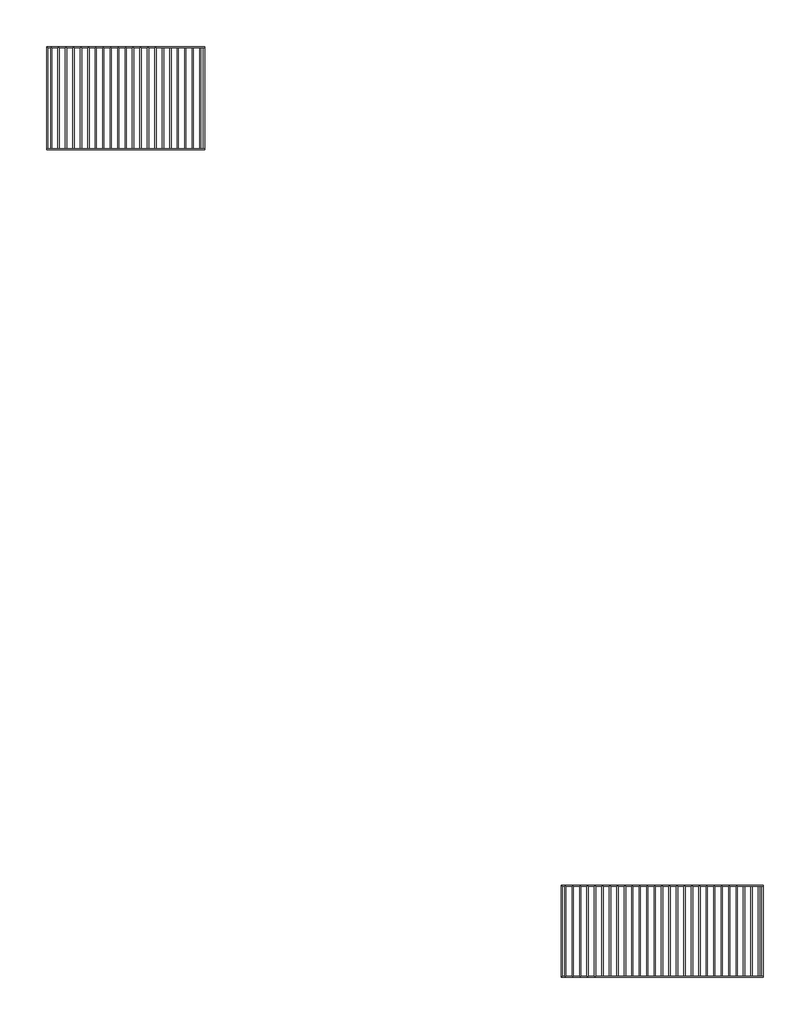
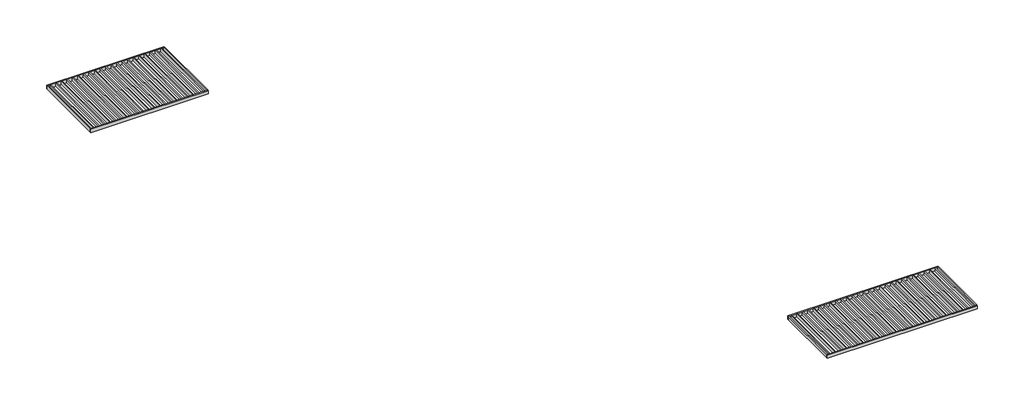
# One storey: 56 beams.
"""IFC4 building model written with IfcOpenShell, lengths in millimetres."""

import ifcopenshell
import ifcopenshell.guid

model = None  # the IFC model being written
_history = None  # IfcOwnerHistory: only IFC2X3 demands one
_inside = {}  # id of a spatial element -> (the spatial element, [elements in it])
_under = {}  # id of a project, library or spatial element -> (it, [spatial elements below it])
_declared = {}  # id of a project -> (the project, [libraries it declares])
_typed = {}  # id of a type object -> (the type object, [elements of that type])
_made_of = {}  # id of a material, layer set ... -> (it, [elements and type objects made of it])


def new_model(schema):
    """Start an empty IFC model of exactly this schema.

    Asked for "IFC4X3", IfcOpenShell would pick the latest addendum, in which some entities
    have other attributes; the version numbers below select the first issue.
    IFC2X3 requires an IfcOwnerHistory on every rooted entity: one is made here for all.
    """
    global model, _history
    if schema == "IFC4X3":
        model = ifcopenshell.file(schema_version=(4, 3, 0, 0))
    else:
        model = ifcopenshell.file(schema=schema)
    _inside.clear()
    _under.clear()
    _declared.clear()
    _typed.clear()
    _made_of.clear()
    _history = None
    if model.schema == "IFC2X3":
        org = make("IfcOrganization", Name="unknown")
        user = make(
            "IfcPersonAndOrganization",
            ThePerson=make("IfcPerson", FamilyName="unknown"),
            TheOrganization=org,
        )
        app = make(
            "IfcApplication",
            ApplicationDeveloper=org,
            Version="unknown",
            ApplicationFullName="unknown",
            ApplicationIdentifier="unknown",
        )
        _history = make(
            "IfcOwnerHistory",
            OwningUser=user,
            OwningApplication=app,
            ChangeAction="ADDED",
            CreationDate=0,
        )
    return model


def make(cls, **values):
    """One entity of the class cls with the attributes given. An attribute that is None is left unset."""
    return model.create_entity(
        cls, **{name: value for name, value in values.items() if value is not None}
    )


def rooted(cls, **values):
    """An entity with a GlobalId (a new one), such as an element, a storey or a relation."""
    return make(cls, GlobalId=ifcopenshell.guid.new(), OwnerHistory=_history, **values)


def si_unit(unit_type, name, prefix=None):
    """IfcSIUnit, for example si_unit("LENGTHUNIT", "METRE", prefix="MILLI")."""
    return make("IfcSIUnit", UnitType=unit_type, Prefix=prefix, Name=name)


def assignment(units):
    """IfcUnitAssignment: the units of a project."""
    return None if units is None else make("IfcUnitAssignment", Units=units)


def point(xyz):
    """IfcCartesianPoint."""
    return None if xyz is None else make("IfcCartesianPoint", Coordinates=xyz)


def direction(xyz):
    """IfcDirection."""
    return None if xyz is None else make("IfcDirection", DirectionRatios=xyz)


def frame(location, z_axis=None, x_axis=None):
    """IfcAxis2Placement3D, a coordinate frame: its origin and axes. An axis left out is left unset."""
    return make(
        "IfcAxis2Placement3D",
        Location=point(location),
        Axis=direction(z_axis),
        RefDirection=direction(x_axis),
    )


def origin():
    """The frame at (0, 0, 0) with its axes left unset."""
    return frame((0.0, 0.0, 0.0))


def place(relative_to, where):
    """IfcLocalPlacement: puts the frame where relative to a parent placement (None: the world)."""
    return make(
        "IfcLocalPlacement", PlacementRelTo=relative_to, RelativePlacement=where
    )


def context(
    kind, dimensions, precision=None, world=None, true_north=None, identifier=None
):
    """IfcGeometricRepresentationContext, for example the 3D "Model" context."""
    return make(
        "IfcGeometricRepresentationContext",
        ContextIdentifier=identifier,
        ContextType=kind,
        CoordinateSpaceDimension=dimensions,
        Precision=precision,
        WorldCoordinateSystem=world,
        TrueNorth=true_north,
    )


def project(units=None, contexts=None):
    """IfcProject with its units and contexts."""
    return rooted(
        "IfcProject",
        Name="project",
        RepresentationContexts=contexts,
        UnitsInContext=assignment(units),
    )


def spatial(cls, under=None, at=None, **own):
    """A site, building, storey or space (cls), placed at a placement, below another one or the project."""
    s = rooted(cls, ObjectPlacement=at, **own)
    if under is not None:
        _under.setdefault(under.id(), (under, []))[1].append(s)
    return s


def polyline(points):
    """IfcPolyline through the points."""
    return make("IfcPolyline", Points=[point(p) for p in points])


def outline(outer, holes=None, kind="AREA"):
    """IfcArbitraryClosedProfileDef: a profile drawn as a closed curve; with holes, ...WithVoids."""
    if holes is None:
        return make("IfcArbitraryClosedProfileDef", ProfileType=kind, OuterCurve=outer)
    return make(
        "IfcArbitraryProfileDefWithVoids",
        ProfileType=kind,
        OuterCurve=outer,
        InnerCurves=holes,
    )


def extrude(swept, where, along, depth):
    """IfcExtrudedAreaSolid: the profile swept, set in the frame where, extruded along a direction by depth."""
    return make(
        "IfcExtrudedAreaSolid",
        SweptArea=swept,
        Position=where,
        ExtrudedDirection=direction(along),
        Depth=depth,
    )


def shape(context_of_items, identifier, shape_type, items):
    """IfcShapeRepresentation: the items that make up one representation, for example the "Body"."""
    return make(
        "IfcShapeRepresentation",
        ContextOfItems=context_of_items,
        RepresentationIdentifier=identifier,
        RepresentationType=shape_type,
        Items=items,
    )


def source(mapping_origin, context_of_items, identifier, shape_type, items):
    """IfcRepresentationMap: a shape defined once, which mapped items show again and again."""
    return make(
        "IfcRepresentationMap",
        MappingOrigin=mapping_origin,
        MappedRepresentation=shape(context_of_items, identifier, shape_type, items),
    )


def transform(
    local_origin,
    x_axis=None,
    y_axis=None,
    z_axis=None,
    scale=None,
    scale2=None,
    scale3=None,
    uniform=True,
):
    """IfcCartesianTransformationOperator3D, or its non-uniform kind. x_axis, y_axis, z_axis: its Axis1, 2, 3."""
    if uniform:
        return make(
            "IfcCartesianTransformationOperator3D",
            Axis1=direction(x_axis),
            Axis2=direction(y_axis),
            LocalOrigin=point(local_origin),
            Scale=scale,
            Axis3=direction(z_axis),
        )
    return make(
        "IfcCartesianTransformationOperator3DnonUniform",
        Axis1=direction(x_axis),
        Axis2=direction(y_axis),
        LocalOrigin=point(local_origin),
        Scale=scale,
        Axis3=direction(z_axis),
        Scale2=scale2,
        Scale3=scale3,
    )


def mapped(mapping_source, mapping_target):
    """IfcMappedItem: shows the shape of a source again, moved by a transform."""
    return make(
        "IfcMappedItem", MappingSource=mapping_source, MappingTarget=mapping_target
    )


def made_of(thing, what):
    """Note that an element or type object is made of a material, layer set ...; save() writes the relation."""
    if what is not None:
        _made_of.setdefault(what.id(), (what, []))[1].append(thing)
    return thing


def element(
    cls,
    number,
    at=None,
    inside=None,
    cuts=None,
    type_object=None,
    material=None,
    context=None,
    identifier="Body",
    shape_type=None,
    held_by="IfcProductDefinitionShape",
    body=None,
    shapes=None,
    **own,
):
    """One element of the class cls, such as IfcWall. Its Tag is "e" and its number.

    at: its placement. inside: the storey or other place that contains it. cuts: it is an
    opening in that element (IfcRelVoidsElement). A single representation is given by context,
    identifier, shape_type and body (its items); several are given by shapes. held_by: the class
    of the entity that holds the representations. save() writes the other relations.
    """
    e = rooted(cls, Tag="e%d" % number, ObjectPlacement=at, **own)
    if body is not None:
        shapes = [shape(context, identifier, shape_type, body)]
    if shapes is not None:
        e.Representation = make(held_by, Representations=shapes)
    if inside is not None:
        _inside.setdefault(inside.id(), (inside, []))[1].append(e)
    if cuts is not None:
        rooted(
            "IfcRelVoidsElement", RelatingBuildingElement=cuts, RelatedOpeningElement=e
        )
    if type_object is not None:
        _typed.setdefault(type_object.id(), (type_object, []))[1].append(e)
    return made_of(e, material)


def aggregate(whole, parts):
    """IfcRelAggregates: a whole, such as a stair, and the parts it consists of."""
    return rooted("IfcRelAggregates", RelatingObject=whole, RelatedObjects=parts)


def save(model, path):
    """Write the relations noted so far, then the file.

    IfcRelAggregates (storeys below a building ...), IfcRelContainedInSpatialStructure (elements
    in a storey), IfcRelDefinesByType, IfcRelAssociatesMaterial and IfcRelDeclares: one each for
    every whole, place, type object, material and project.
    """
    for whole, parts in _under.values():
        aggregate(whole, parts)
    for where, things in _inside.values():
        rooted(
            "IfcRelContainedInSpatialStructure",
            RelatedElements=things,
            RelatingStructure=where,
        )
    for kind, things in _typed.values():
        rooted("IfcRelDefinesByType", RelatedObjects=things, RelatingType=kind)
    for what, things in _made_of.values():
        rooted("IfcRelAssociatesMaterial", RelatedObjects=things, RelatingMaterial=what)
    for by, libraries in _declared.values():
        rooted("IfcRelDeclares", RelatingContext=by, RelatedDefinitions=libraries)
    model.write(path)


def beam_80e5a63c(model_context):
    return source(origin(), model_context, "Body", "SweptSolid", [
        extrude(outline(polyline([(-2451.0, -35.0), (-2451.0, 35.0), (2451.0, 35.0), (2451.0, -35.0), (-2451.0, -35.0)])), frame((0.0, 0.0, -122.5), z_axis=(0.0, 0.0, 1.0), x_axis=(1.0, 0.0, 0.0)), (0.0, 0.0, 1.0), 245.0),
    ])


def beam_9365c9be(model_context):
    return source(origin(), model_context, "Body", "SweptSolid", [
        extrude(outline(polyline([(-2751.0, -35.0), (-2751.0, 35.0), (2751.0, 35.0), (2751.0, -35.0), (-2751.0, -35.0)])), frame((0.0, 0.0, -122.5), z_axis=(0.0, 0.0, 1.0), x_axis=(1.0, 0.0, 0.0)), (0.0, 0.0, 1.0), 245.0),
    ])


model = new_model("IFC4")

# Units and contexts
model_context = context("Model", 3, world=origin())
ifc_project = project(units=[si_unit("LENGTHUNIT", "METRE", prefix="MILLI")], contexts=[model_context])

# Site, building, storey
site = spatial("IfcSite", under=ifc_project)
building = spatial("IfcBuilding", under=site)
storey = spatial("IfcBuildingStorey", under=building, Name="03c_bk balklaag installatieopbouw", Elevation=15500.0)

# Beams
placement = place(None, origin())
element("IfcBeam", 1, ObjectType="NLRS_28_SF_LIB_houten balk-MMBW-SRP_gen_rsf : houten balk_gen__bxh 70x195", at=placement, inside=storey, context=model_context, shape_type="SweptSolid", body=[
    extrude(outline(polyline([(64806.0, 5201.0), (64876.0, 5201.0), (64876.0, 299.0), (64806.0, 299.0), (64806.0, 5201.0)])), frame((0.0, 0.0, 15255.0), z_axis=(0.0, 0.0, 1.0), x_axis=(1.0, 0.0, 0.0)), (0.0, 0.0, 1.0), 245.0),
])
element("IfcBeam", 2, ObjectType="NLRS_28_SF_LIB_houten balk-MMBW-SRP_gen_rsf : houten balk_gen__bxh 70x195", at=placement, inside=storey, context=model_context, shape_type="SweptSolid", body=[
    extrude(outline(polyline([(64399.0, 5201.0), (64469.0, 5201.0), (64469.0, 299.0), (64399.0, 299.0), (64399.0, 5201.0)])), frame((0.0, 0.0, 15255.0), z_axis=(0.0, 0.0, 1.0), x_axis=(1.0, 0.0, 0.0)), (0.0, 0.0, 1.0), 245.0),
])
element("IfcBeam", 3, ObjectType="NLRS_28_SF_LIB_houten balk-MMBW-SRP_gen_rsf : houten balk_gen__bxh 70x195", at=placement, inside=storey, context=model_context, shape_type="SweptSolid", body=[
    extrude(outline(polyline([(63992.0, 5201.0), (64062.0, 5201.0), (64062.0, 299.0), (63992.0, 299.0), (63992.0, 5201.0)])), frame((0.0, 0.0, 15255.0), z_axis=(0.0, 0.0, 1.0), x_axis=(1.0, 0.0, 0.0)), (0.0, 0.0, 1.0), 245.0),
])
element("IfcBeam", 4, ObjectType="NLRS_28_SF_LIB_houten balk-MMBW-SRP_gen_rsf : houten balk_gen__bxh 70x195", at=placement, inside=storey, context=model_context, shape_type="SweptSolid", body=[
    extrude(outline(polyline([(63585.0, 5201.0), (63655.0, 5201.0), (63655.0, 299.0), (63585.0, 299.0), (63585.0, 5201.0)])), frame((0.0, 0.0, 15255.0), z_axis=(0.0, 0.0, 1.0), x_axis=(1.0, 0.0, 0.0)), (0.0, 0.0, 1.0), 245.0),
])
element("IfcBeam", 5, ObjectType="NLRS_28_SF_LIB_houten balk-MMBW-SRP_gen_rsf : houten balk_gen__bxh 70x195", at=placement, inside=storey, context=model_context, shape_type="SweptSolid", body=[
    extrude(outline(polyline([(63178.0, 5201.0), (63248.0, 5201.0), (63248.0, 299.0), (63178.0, 299.0), (63178.0, 5201.0)])), frame((0.0, 0.0, 15255.0), z_axis=(0.0, 0.0, 1.0), x_axis=(1.0, 0.0, 0.0)), (0.0, 0.0, 1.0), 245.0),
])
element("IfcBeam", 6, ObjectType="NLRS_28_SF_LIB_houten balk-MMBW-SRP_gen_rsf : houten balk_gen__bxh 70x195", at=placement, inside=storey, context=model_context, shape_type="SweptSolid", body=[
    extrude(outline(polyline([(62771.0, 5201.0), (62841.0, 5201.0), (62841.0, 299.0), (62771.0, 299.0), (62771.0, 5201.0)])), frame((0.0, 0.0, 15255.0), z_axis=(0.0, 0.0, 1.0), x_axis=(1.0, 0.0, 0.0)), (0.0, 0.0, 1.0), 245.0),
])
element("IfcBeam", 7, ObjectType="NLRS_28_SF_LIB_houten balk-MMBW-SRP_gen_rsf : houten balk_gen__bxh 70x195", at=placement, inside=storey, context=model_context, shape_type="SweptSolid", body=[
    extrude(outline(polyline([(62364.0, 5201.0), (62434.0, 5201.0), (62434.0, 299.0), (62364.0, 299.0), (62364.0, 5201.0)])), frame((0.0, 0.0, 15255.0), z_axis=(0.0, 0.0, 1.0), x_axis=(1.0, 0.0, 0.0)), (0.0, 0.0, 1.0), 245.0),
])
element("IfcBeam", 8, ObjectType="NLRS_28_SF_LIB_houten balk-MMBW-SRP_gen_rsf : houten balk_gen__bxh 70x195", at=placement, inside=storey, context=model_context, shape_type="SweptSolid", body=[
    extrude(outline(polyline([(61957.0, 5201.0), (62027.0, 5201.0), (62027.0, 299.0), (61957.0, 299.0), (61957.0, 5201.0)])), frame((0.0, 0.0, 15255.0), z_axis=(0.0, 0.0, 1.0), x_axis=(1.0, 0.0, 0.0)), (0.0, 0.0, 1.0), 245.0),
])
element("IfcBeam", 9, ObjectType="NLRS_28_SF_LIB_houten balk-MMBW-SRP_gen_rsf : houten balk_gen__bxh 70x195", at=placement, inside=storey, context=model_context, shape_type="SweptSolid", body=[
    extrude(outline(polyline([(61550.0, 5201.0), (61620.0, 5201.0), (61620.0, 299.0), (61550.0, 299.0), (61550.0, 5201.0)])), frame((0.0, 0.0, 15255.0), z_axis=(0.0, 0.0, 1.0), x_axis=(1.0, 0.0, 0.0)), (0.0, 0.0, 1.0), 245.0),
])
element("IfcBeam", 10, ObjectType="NLRS_28_SF_LIB_houten balk-MMBW-SRP_gen_rsf : houten balk_gen__bxh 70x195", at=placement, inside=storey, context=model_context, shape_type="SweptSolid", body=[
    extrude(outline(polyline([(61143.0, 5201.0), (61213.0, 5201.0), (61213.0, 299.0), (61143.0, 299.0), (61143.0, 5201.0)])), frame((0.0, 0.0, 15255.0), z_axis=(0.0, 0.0, 1.0), x_axis=(1.0, 0.0, 0.0)), (0.0, 0.0, 1.0), 245.0),
])
element("IfcBeam", 11, ObjectType="NLRS_28_SF_LIB_houten balk-MMBW-SRP_gen_rsf : houten balk_gen__bxh 70x195", at=placement, inside=storey, context=model_context, shape_type="SweptSolid", body=[
    extrude(outline(polyline([(60736.0, 5201.0), (60806.0, 5201.0), (60806.0, 299.0), (60736.0, 299.0), (60736.0, 5201.0)])), frame((0.0, 0.0, 15255.0), z_axis=(0.0, 0.0, 1.0), x_axis=(1.0, 0.0, 0.0)), (0.0, 0.0, 1.0), 245.0),
])
element("IfcBeam", 12, ObjectType="NLRS_28_SF_LIB_houten balk-MMBW-SRP_gen_rsf : houten balk_gen__bxh 70x195", at=placement, inside=storey, context=model_context, shape_type="SweptSolid", body=[
    extrude(outline(polyline([(60329.0, 5201.0), (60399.0, 5201.0), (60399.0, 299.0), (60329.0, 299.0), (60329.0, 5201.0)])), frame((0.0, 0.0, 15255.0), z_axis=(0.0, 0.0, 1.0), x_axis=(1.0, 0.0, 0.0)), (0.0, 0.0, 1.0), 245.0),
])
element("IfcBeam", 13, ObjectType="NLRS_28_SF_LIB_houten balk-MMBW-SRP_gen_rsf : houten balk_gen__bxh 70x195", at=placement, inside=storey, context=model_context, shape_type="SweptSolid", body=[
    extrude(outline(polyline([(59922.0, 5201.0), (59992.0, 5201.0), (59992.0, 299.0), (59922.0, 299.0), (59922.0, 5201.0)])), frame((0.0, 0.0, 15255.0), z_axis=(0.0, 0.0, 1.0), x_axis=(1.0, 0.0, 0.0)), (0.0, 0.0, 1.0), 245.0),
])
element("IfcBeam", 14, ObjectType="NLRS_28_SF_LIB_houten balk-MMBW-SRP_gen_rsf : houten balk_gen__bxh 70x195", at=placement, inside=storey, context=model_context, shape_type="SweptSolid", body=[
    extrude(outline(polyline([(59515.0, 5201.0), (59585.0, 5201.0), (59585.0, 299.0), (59515.0, 299.0), (59515.0, 5201.0)])), frame((0.0, 0.0, 15255.0), z_axis=(0.0, 0.0, 1.0), x_axis=(1.0, 0.0, 0.0)), (0.0, 0.0, 1.0), 245.0),
])
element("IfcBeam", 15, ObjectType="NLRS_28_SF_LIB_houten balk-MMBW-SRP_gen_rsf : houten balk_gen__bxh 70x195", at=placement, inside=storey, context=model_context, shape_type="SweptSolid", body=[
    extrude(outline(polyline([(59108.0, 5201.0), (59178.0, 5201.0), (59178.0, 299.0), (59108.0, 299.0), (59108.0, 5201.0)])), frame((0.0, 0.0, 15255.0), z_axis=(0.0, 0.0, 1.0), x_axis=(1.0, 0.0, 0.0)), (0.0, 0.0, 1.0), 245.0),
])
element("IfcBeam", 16, ObjectType="NLRS_28_SF_LIB_houten balk-MMBW-SRP_gen_rsf : houten balk_gen__bxh 70x195", at=placement, inside=storey, context=model_context, shape_type="SweptSolid", body=[
    extrude(outline(polyline([(58701.0, 5201.0), (58771.0, 5201.0), (58771.0, 299.0), (58701.0, 299.0), (58701.0, 5201.0)])), frame((0.0, 0.0, 15255.0), z_axis=(0.0, 0.0, 1.0), x_axis=(1.0, 0.0, 0.0)), (0.0, 0.0, 1.0), 245.0),
])
element("IfcBeam", 17, ObjectType="NLRS_28_SF_LIB_houten balk-MMBW-SRP_gen_rsf : houten balk_gen__bxh 70x195", at=placement, inside=storey, context=model_context, shape_type="SweptSolid", body=[
    extrude(outline(polyline([(58294.0, 5201.0), (58364.0, 5201.0), (58364.0, 299.0), (58294.0, 299.0), (58294.0, 5201.0)])), frame((0.0, 0.0, 15255.0), z_axis=(0.0, 0.0, 1.0), x_axis=(1.0, 0.0, 0.0)), (0.0, 0.0, 1.0), 245.0),
])
element("IfcBeam", 18, ObjectType="NLRS_28_SF_LIB_houten balk-MMBW-SRP_gen_rsf : houten balk_gen__bxh 70x195", at=placement, inside=storey, context=model_context, shape_type="SweptSolid", body=[
    extrude(outline(polyline([(57887.0, 5201.0), (57957.0, 5201.0), (57957.0, 299.0), (57887.0, 299.0), (57887.0, 5201.0)])), frame((0.0, 0.0, 15255.0), z_axis=(0.0, 0.0, 1.0), x_axis=(1.0, 0.0, 0.0)), (0.0, 0.0, 1.0), 245.0),
])
element("IfcBeam", 19, ObjectType="NLRS_28_SF_LIB_houten balk-MMBW-SRP_gen_rsf : houten balk_gen__bxh 70x195", at=placement, inside=storey, context=model_context, shape_type="SweptSolid", body=[
    extrude(outline(polyline([(57480.0, 5201.0), (57550.0, 5201.0), (57550.0, 299.0), (57480.0, 299.0), (57480.0, 5201.0)])), frame((0.0, 0.0, 15255.0), z_axis=(0.0, 0.0, 1.0), x_axis=(1.0, 0.0, 0.0)), (0.0, 0.0, 1.0), 245.0),
])
element("IfcBeam", 20, ObjectType="NLRS_28_SF_LIB_houten balk-MMBW-SRP_gen_rsf : houten balk_gen__bxh 70x195", at=placement, inside=storey, context=model_context, shape_type="SweptSolid", body=[
    extrude(outline(polyline([(34285.0, 51001.0), (34355.0, 51001.0), (34355.0, 45499.0), (34285.0, 45499.0), (34285.0, 51001.0)])), frame((0.0, 0.0, 15255.0), z_axis=(0.0, 0.0, 1.0), x_axis=(1.0, 0.0, 0.0)), (0.0, 0.0, 1.0), 245.0),
])
element("IfcBeam", 21, ObjectType="NLRS_28_SF_LIB_houten balk-MMBW-SRP_gen_rsf : houten balk_gen__bxh 70x195", at=placement, inside=storey, context=model_context, shape_type="SweptSolid", body=[
    extrude(outline(polyline([(33878.0, 51001.0), (33948.0, 51001.0), (33948.0, 45499.0), (33878.0, 45499.0), (33878.0, 51001.0)])), frame((0.0, 0.0, 15255.0), z_axis=(0.0, 0.0, 1.0), x_axis=(1.0, 0.0, 0.0)), (0.0, 0.0, 1.0), 245.0),
])
element("IfcBeam", 22, ObjectType="NLRS_28_SF_LIB_houten balk-MMBW-SRP_gen_rsf : houten balk_gen__bxh 70x195", at=placement, inside=storey, context=model_context, shape_type="SweptSolid", body=[
    extrude(outline(polyline([(33471.0, 51001.0), (33541.0, 51001.0), (33541.0, 45499.0), (33471.0, 45499.0), (33471.0, 51001.0)])), frame((0.0, 0.0, 15255.0), z_axis=(0.0, 0.0, 1.0), x_axis=(1.0, 0.0, 0.0)), (0.0, 0.0, 1.0), 245.0),
])
element("IfcBeam", 23, ObjectType="NLRS_28_SF_LIB_houten balk-MMBW-SRP_gen_rsf : houten balk_gen__bxh 70x195", at=placement, inside=storey, context=model_context, shape_type="SweptSolid", body=[
    extrude(outline(polyline([(33064.0, 51001.0), (33134.0, 51001.0), (33134.0, 45499.0), (33064.0, 45499.0), (33064.0, 51001.0)])), frame((0.0, 0.0, 15255.0), z_axis=(0.0, 0.0, 1.0), x_axis=(1.0, 0.0, 0.0)), (0.0, 0.0, 1.0), 245.0),
])
element("IfcBeam", 24, ObjectType="NLRS_28_SF_LIB_houten balk-MMBW-SRP_gen_rsf : houten balk_gen__bxh 70x195", at=placement, inside=storey, context=model_context, shape_type="SweptSolid", body=[
    extrude(outline(polyline([(32657.0, 51001.0), (32727.0, 51001.0), (32727.0, 45499.0), (32657.0, 45499.0), (32657.0, 51001.0)])), frame((0.0, 0.0, 15255.0), z_axis=(0.0, 0.0, 1.0), x_axis=(1.0, 0.0, 0.0)), (0.0, 0.0, 1.0), 245.0),
])
element("IfcBeam", 25, ObjectType="NLRS_28_SF_LIB_houten balk-MMBW-SRP_gen_rsf : houten balk_gen__bxh 70x195", at=placement, inside=storey, context=model_context, shape_type="SweptSolid", body=[
    extrude(outline(polyline([(32250.0, 51001.0), (32320.0, 51001.0), (32320.0, 45499.0), (32250.0, 45499.0), (32250.0, 51001.0)])), frame((0.0, 0.0, 15255.0), z_axis=(0.0, 0.0, 1.0), x_axis=(1.0, 0.0, 0.0)), (0.0, 0.0, 1.0), 245.0),
])
element("IfcBeam", 26, ObjectType="NLRS_28_SF_LIB_houten balk-MMBW-SRP_gen_rsf : houten balk_gen__bxh 70x195", at=placement, inside=storey, context=model_context, shape_type="SweptSolid", body=[
    extrude(outline(polyline([(31843.0, 51001.0), (31913.0, 51001.0), (31913.0, 45499.0), (31843.0, 45499.0), (31843.0, 51001.0)])), frame((0.0, 0.0, 15255.0), z_axis=(0.0, 0.0, 1.0), x_axis=(1.0, 0.0, 0.0)), (0.0, 0.0, 1.0), 245.0),
])
element("IfcBeam", 27, ObjectType="NLRS_28_SF_LIB_houten balk-MMBW-SRP_gen_rsf : houten balk_gen__bxh 70x195", at=placement, inside=storey, context=model_context, shape_type="SweptSolid", body=[
    extrude(outline(polyline([(31436.0, 51001.0), (31506.0, 51001.0), (31506.0, 45499.0), (31436.0, 45499.0), (31436.0, 51001.0)])), frame((0.0, 0.0, 15255.0), z_axis=(0.0, 0.0, 1.0), x_axis=(1.0, 0.0, 0.0)), (0.0, 0.0, 1.0), 245.0),
])
element("IfcBeam", 28, ObjectType="NLRS_28_SF_LIB_houten balk-MMBW-SRP_gen_rsf : houten balk_gen__bxh 70x195", at=placement, inside=storey, context=model_context, shape_type="SweptSolid", body=[
    extrude(outline(polyline([(31029.0, 51001.0), (31099.0, 51001.0), (31099.0, 45499.0), (31029.0, 45499.0), (31029.0, 51001.0)])), frame((0.0, 0.0, 15255.0), z_axis=(0.0, 0.0, 1.0), x_axis=(1.0, 0.0, 0.0)), (0.0, 0.0, 1.0), 245.0),
])
element("IfcBeam", 29, ObjectType="NLRS_28_SF_LIB_houten balk-MMBW-SRP_gen_rsf : houten balk_gen__bxh 70x195", at=placement, inside=storey, context=model_context, shape_type="SweptSolid", body=[
    extrude(outline(polyline([(30622.0, 51001.0), (30692.0, 51001.0), (30692.0, 45499.0), (30622.0, 45499.0), (30622.0, 51001.0)])), frame((0.0, 0.0, 15255.0), z_axis=(0.0, 0.0, 1.0), x_axis=(1.0, 0.0, 0.0)), (0.0, 0.0, 1.0), 245.0),
])
element("IfcBeam", 30, ObjectType="NLRS_28_SF_LIB_houten balk-MMBW-SRP_gen_rsf : houten balk_gen__bxh 70x195", at=placement, inside=storey, context=model_context, shape_type="SweptSolid", body=[
    extrude(outline(polyline([(30215.0, 51001.0), (30285.0, 51001.0), (30285.0, 45499.0), (30215.0, 45499.0), (30215.0, 51001.0)])), frame((0.0, 0.0, 15255.0), z_axis=(0.0, 0.0, 1.0), x_axis=(1.0, 0.0, 0.0)), (0.0, 0.0, 1.0), 245.0),
])
element("IfcBeam", 31, ObjectType="NLRS_28_SF_LIB_houten balk-MMBW-SRP_gen_rsf : houten balk_gen__bxh 70x195", at=placement, inside=storey, context=model_context, shape_type="SweptSolid", body=[
    extrude(outline(polyline([(29808.0, 51001.0), (29878.0, 51001.0), (29878.0, 45499.0), (29808.0, 45499.0), (29808.0, 51001.0)])), frame((0.0, 0.0, 15255.0), z_axis=(0.0, 0.0, 1.0), x_axis=(1.0, 0.0, 0.0)), (0.0, 0.0, 1.0), 245.0),
])
element("IfcBeam", 32, ObjectType="NLRS_28_SF_LIB_houten balk-MMBW-SRP_gen_rsf : houten balk_gen__bxh 70x195", at=placement, inside=storey, context=model_context, shape_type="SweptSolid", body=[
    extrude(outline(polyline([(29401.0, 51001.0), (29471.0, 51001.0), (29471.0, 45499.0), (29401.0, 45499.0), (29401.0, 51001.0)])), frame((0.0, 0.0, 15255.0), z_axis=(0.0, 0.0, 1.0), x_axis=(1.0, 0.0, 0.0)), (0.0, 0.0, 1.0), 245.0),
])
element("IfcBeam", 33, ObjectType="NLRS_28_SF_LIB_houten balk-MMBW-SRP_gen_rsf : houten balk_gen__bxh 70x195", at=placement, inside=storey, context=model_context, shape_type="SweptSolid", body=[
    extrude(outline(polyline([(28994.0, 51001.0), (29064.0, 51001.0), (29064.0, 45499.0), (28994.0, 45499.0), (28994.0, 51001.0)])), frame((0.0, 0.0, 15255.0), z_axis=(0.0, 0.0, 1.0), x_axis=(1.0, 0.0, 0.0)), (0.0, 0.0, 1.0), 245.0),
])
element("IfcBeam", 34, ObjectType="NLRS_28_SF_LIB_houten balk-MMBW-SRP_gen_rsf : houten balk_gen__bxh 70x195", at=placement, inside=storey, context=model_context, shape_type="SweptSolid", body=[
    extrude(outline(polyline([(28587.0, 51001.0), (28657.0, 51001.0), (28657.0, 45499.0), (28587.0, 45499.0), (28587.0, 51001.0)])), frame((0.0, 0.0, 15255.0), z_axis=(0.0, 0.0, 1.0), x_axis=(1.0, 0.0, 0.0)), (0.0, 0.0, 1.0), 245.0),
])
element("IfcBeam", 35, ObjectType="NLRS_28_SF_LIB_houten balk-MMBW-SRP_gen_rsf : houten balk_gen__bxh 70x195", at=placement, inside=storey, context=model_context, shape_type="SweptSolid", body=[
    extrude(outline(polyline([(65001.0, 5188.3), (65071.0, 5188.3), (65071.0, 311.7), (65001.0, 311.7), (65001.0, 5188.3)])), frame((0.0, 0.0, 15255.0), z_axis=(0.0, 0.0, 1.0), x_axis=(1.0, 0.0, 0.0)), (0.0, 0.0, 1.0), 245.0),
])
element("IfcBeam", 36, ObjectType="NLRS_28_SF_LIB_houten balk-MMBW-SRP_gen_rsf : houten balk_gen__bxh 70x195", at=placement, inside=storey, context=model_context, shape_type="SweptSolid", body=[
    extrude(outline(polyline([(54029.0, 5201.0), (54099.0, 5201.0), (54099.0, 299.0), (54029.0, 299.0), (54029.0, 5201.0)])), frame((0.0, 0.0, 15255.0), z_axis=(0.0, 0.0, 1.0), x_axis=(1.0, 0.0, 0.0)), (0.0, 0.0, 1.0), 245.0),
])
element("IfcBeam", 37, ObjectType="NLRS_28_SF_LIB_houten balk-MMBW-SRP_gen_rsf : houten balk_gen__bxh 70x195", at=placement, inside=storey, context=model_context, shape_type="SweptSolid", body=[
    extrude(outline(polyline([(25929.0, 51001.0), (25999.0, 51001.0), (25999.0, 45499.0), (25929.0, 45499.0), (25929.0, 51001.0)])), frame((0.0, 0.0, 15255.0), z_axis=(0.0, 0.0, 1.0), x_axis=(1.0, 0.0, 0.0)), (0.0, 0.0, 1.0), 245.0),
])
element("IfcBeam", 38, ObjectType="NLRS_28_SF_LIB_houten balk-MMBW-SRP_gen_rsf : houten balk_gen__bxh 70x195", at=placement, inside=storey, context=model_context, shape_type="SweptSolid", body=[
    extrude(outline(polyline([(34501.0, 51001.0), (34571.0, 51001.0), (34571.0, 45499.0), (34501.0, 45499.0), (34501.0, 51001.0)])), frame((0.0, 0.0, 15255.0), z_axis=(0.0, 0.0, 1.0), x_axis=(1.0, 0.0, 0.0)), (0.0, 0.0, 1.0), 245.0),
])
element("IfcBeam", 39, ObjectType="NLRS_28_SF_LIB_houten balk-MMBW-SRP_gen_rsf : houten balk_gen__bxh 70x195", at=placement, inside=storey, context=model_context, shape_type="SweptSolid", body=[
    extrude(outline(polyline([(65071.0, 299.0), (65071.0, 229.0), (54029.0, 229.0), (54029.0, 299.0), (65071.0, 299.0)])), frame((0.0, 0.0, 15255.0), z_axis=(0.0, 0.0, 1.0), x_axis=(1.0, 0.0, 0.0)), (0.0, 0.0, 1.0), 245.0),
])
element("IfcBeam", 40, ObjectType="NLRS_28_SF_LIB_houten balk-MMBW-SRP_gen_rsf : houten balk_gen__bxh 70x195", at=placement, inside=storey, context=model_context, shape_type="SweptSolid", body=[
    extrude(outline(polyline([(65071.0, 5271.0), (65071.0, 5201.0), (54029.0, 5201.0), (54029.0, 5271.0), (65071.0, 5271.0)])), frame((0.0, 0.0, 15255.0), z_axis=(0.0, 0.0, 1.0), x_axis=(1.0, 0.0, 0.0)), (0.0, 0.0, 1.0), 245.0),
])
element("IfcBeam", 41, ObjectType="NLRS_28_SF_LIB_houten balk-MMBW-SRP_gen_rsf : houten balk_gen__bxh 70x195", at=placement, inside=storey, context=model_context, shape_type="SweptSolid", body=[
    extrude(outline(polyline([(34571.0, 45499.0), (34571.0, 45429.0), (25929.0, 45429.0), (25929.0, 45499.0), (34571.0, 45499.0)])), frame((0.0, 0.0, 15255.0), z_axis=(0.0, 0.0, 1.0), x_axis=(1.0, 0.0, 0.0)), (0.0, 0.0, 1.0), 245.0),
])
element("IfcBeam", 42, ObjectType="NLRS_28_SF_LIB_houten balk-MMBW-SRP_gen_rsf : houten balk_gen__bxh 70x195", at=placement, inside=storey, context=model_context, shape_type="SweptSolid", body=[
    extrude(outline(polyline([(34571.0, 51071.0), (34571.0, 51001.0), (25929.0, 51001.0), (25929.0, 51071.0), (34571.0, 51071.0)])), frame((0.0, 0.0, 15255.0), z_axis=(0.0, 0.0, 1.0), x_axis=(1.0, 0.0, 0.0)), (0.0, 0.0, 1.0), 245.0),
])
beam_shape = beam_80e5a63c(model_context)
element("IfcBeam", 43, ObjectType="NLRS_28_SF_LIB_houten balk-MMBW-SRP_gen_rsf : houten balk_gen__bxh 70x195", at=placement, inside=storey, context=model_context, shape_type="MappedRepresentation", body=[
    mapped(beam_shape, transform((57108.0, 2750.0, 15377.5), x_axis=(0.0, -1.0, 0.0), y_axis=(1.0, 0.0, 0.0), z_axis=(0.0, 0.0, 1.0))),
])
element("IfcBeam", 44, ObjectType="NLRS_28_SF_LIB_houten balk-MMBW-SRP_gen_rsf : houten balk_gen__bxh 70x195", at=placement, inside=storey, context=model_context, shape_type="MappedRepresentation", body=[
    mapped(beam_shape, transform((56701.0, 2750.0, 15377.5), x_axis=(0.0, -1.0, 0.0), y_axis=(1.0, 0.0, 0.0), z_axis=(0.0, 0.0, 1.0))),
])
element("IfcBeam", 45, ObjectType="NLRS_28_SF_LIB_houten balk-MMBW-SRP_gen_rsf : houten balk_gen__bxh 70x195", at=placement, inside=storey, context=model_context, shape_type="MappedRepresentation", body=[
    mapped(beam_shape, transform((56294.0, 2750.0, 15377.5), x_axis=(0.0, -1.0, 0.0), y_axis=(1.0, 0.0, 0.0), z_axis=(0.0, 0.0, 1.0))),
])
element("IfcBeam", 46, ObjectType="NLRS_28_SF_LIB_houten balk-MMBW-SRP_gen_rsf : houten balk_gen__bxh 70x195", at=placement, inside=storey, context=model_context, shape_type="MappedRepresentation", body=[
    mapped(beam_shape, transform((55887.0, 2750.0, 15377.5), x_axis=(0.0, -1.0, 0.0), y_axis=(1.0, 0.0, 0.0), z_axis=(0.0, 0.0, 1.0))),
])
element("IfcBeam", 47, ObjectType="NLRS_28_SF_LIB_houten balk-MMBW-SRP_gen_rsf : houten balk_gen__bxh 70x195", at=placement, inside=storey, context=model_context, shape_type="MappedRepresentation", body=[
    mapped(beam_shape, transform((55480.0, 2750.0, 15377.5), x_axis=(0.0, -1.0, 0.0), y_axis=(1.0, 0.0, 0.0), z_axis=(0.0, 0.0, 1.0))),
])
element("IfcBeam", 48, ObjectType="NLRS_28_SF_LIB_houten balk-MMBW-SRP_gen_rsf : houten balk_gen__bxh 70x195", at=placement, inside=storey, context=model_context, shape_type="MappedRepresentation", body=[
    mapped(beam_shape, transform((55073.0, 2750.0, 15377.5), x_axis=(0.0, -1.0, 0.0), y_axis=(1.0, 0.0, 0.0), z_axis=(0.0, 0.0, 1.0))),
])
element("IfcBeam", 49, ObjectType="NLRS_28_SF_LIB_houten balk-MMBW-SRP_gen_rsf : houten balk_gen__bxh 70x195", at=placement, inside=storey, context=model_context, shape_type="MappedRepresentation", body=[
    mapped(beam_shape, transform((54666.0, 2750.0, 15377.5), x_axis=(0.0, -1.0, 0.0), y_axis=(1.0, 0.0, 0.0), z_axis=(0.0, 0.0, 1.0))),
])
element("IfcBeam", 50, ObjectType="NLRS_28_SF_LIB_houten balk-MMBW-SRP_gen_rsf : houten balk_gen__bxh 70x195", at=placement, inside=storey, context=model_context, shape_type="MappedRepresentation", body=[
    mapped(beam_shape, transform((54259.0, 2750.0, 15377.5), x_axis=(0.0, -1.0, 0.0), y_axis=(1.0, 0.0, 0.0), z_axis=(0.0, 0.0, 1.0))),
])
beam_2_shape = beam_9365c9be(model_context)
element("IfcBeam", 51, ObjectType="NLRS_28_SF_LIB_houten balk-MMBW-SRP_gen_rsf : houten balk_gen__bxh 70x195", at=placement, inside=storey, context=model_context, shape_type="MappedRepresentation", body=[
    mapped(beam_2_shape, transform((28215.0, 48250.0, 15377.5), x_axis=(0.0, -1.0, 0.0), y_axis=(1.0, 0.0, 0.0), z_axis=(0.0, 0.0, 1.0))),
])
element("IfcBeam", 52, ObjectType="NLRS_28_SF_LIB_houten balk-MMBW-SRP_gen_rsf : houten balk_gen__bxh 70x195", at=placement, inside=storey, context=model_context, shape_type="MappedRepresentation", body=[
    mapped(beam_2_shape, transform((27808.0, 48250.0, 15377.5), x_axis=(0.0, -1.0, 0.0), y_axis=(1.0, 0.0, 0.0), z_axis=(0.0, 0.0, 1.0))),
])
element("IfcBeam", 53, ObjectType="NLRS_28_SF_LIB_houten balk-MMBW-SRP_gen_rsf : houten balk_gen__bxh 70x195", at=placement, inside=storey, context=model_context, shape_type="MappedRepresentation", body=[
    mapped(beam_2_shape, transform((27401.0, 48250.0, 15377.5), x_axis=(0.0, -1.0, 0.0), y_axis=(1.0, 0.0, 0.0), z_axis=(0.0, 0.0, 1.0))),
])
element("IfcBeam", 54, ObjectType="NLRS_28_SF_LIB_houten balk-MMBW-SRP_gen_rsf : houten balk_gen__bxh 70x195", at=placement, inside=storey, context=model_context, shape_type="MappedRepresentation", body=[
    mapped(beam_2_shape, transform((26994.0, 48250.0, 15377.5), x_axis=(0.0, -1.0, 0.0), y_axis=(1.0, 0.0, 0.0), z_axis=(0.0, 0.0, 1.0))),
])
element("IfcBeam", 55, ObjectType="NLRS_28_SF_LIB_houten balk-MMBW-SRP_gen_rsf : houten balk_gen__bxh 70x195", at=placement, inside=storey, context=model_context, shape_type="MappedRepresentation", body=[
    mapped(beam_2_shape, transform((26587.0, 48250.0, 15377.5), x_axis=(0.0, -1.0, 0.0), y_axis=(1.0, 0.0, 0.0), z_axis=(0.0, 0.0, 1.0))),
])
element("IfcBeam", 56, ObjectType="NLRS_28_SF_LIB_houten balk-MMBW-SRP_gen_rsf : houten balk_gen__bxh 70x195", at=placement, inside=storey, context=model_context, shape_type="MappedRepresentation", body=[
    mapped(beam_2_shape, transform((26180.0, 48250.0, 15377.5), x_axis=(0.0, -1.0, 0.0), y_axis=(1.0, 0.0, 0.0), z_axis=(0.0, 0.0, 1.0))),
])

save(model, "model.ifc")

# Revit data of these elements
# Type "NLRS_28_SF_LIB_houten balk-MMBW-SRP_gen_rsf : houten balk_gen__bxh 70x195"
#   Type IfcGUID = "07M7mRoiH1CR8m_RSKIvYS"
#   IfcExportAs = "IfcBeamType"
#   Type Comments = "70x195"
#   Model = " "
#   Manufacturer = " "
#   Fire Rating = " "
#   Description = "houten balk 70x195"
#   Assembly Code = "28.11"
#   NLRS_C_lengte [instance default] = 3000 mm
#   NLRS_C_hoogte = 245 mm
#   NLRS_C_breedte = 70 mm
#   Length [instance default] = 3000 mm
#   Structural Material = NLRS_i2_hout naaldhout vuren_gen_rsf
#   Keynote = ""
# Element 1 (IfcBeam, "NLRS_28_SF_LIB_houten balk-MMBW-SRP_gen_rsf : houten balk_gen__bxh 70x195")
#   IfcGUID = "07M7mRoiH1CR8m_RSKIwKW"
#   NLRS_C_lengte = 4972 mm
#   IsExternal = yes
#   LoadBearing = yes
#   Phase Created = NLRS_nieuw
#   Materials on its faces: "NLRS_i2_hout naaldhout vuren_gen_rsf"
# Element 2 (IfcBeam, "NLRS_28_SF_LIB_houten balk-MMBW-SRP_gen_rsf : houten balk_gen__bxh 70x195")
#   IfcGUID = "07M7mRoiH1CR8m_RSKIwKc"
#   NLRS_C_lengte = 4972 mm
#   IsExternal = yes
#   LoadBearing = yes
#   Phase Created = NLRS_nieuw
#   Materials on its faces: "NLRS_i2_hout naaldhout vuren_gen_rsf"
# Element 3 (IfcBeam, "NLRS_28_SF_LIB_houten balk-MMBW-SRP_gen_rsf : houten balk_gen__bxh 70x195")
#   IfcGUID = "07M7mRoiH1CR8m_RSKIwKa"
#   NLRS_C_lengte = 4972 mm
#   IsExternal = yes
#   LoadBearing = yes
#   Phase Created = NLRS_nieuw
#   Materials on its faces: "NLRS_i2_hout naaldhout vuren_gen_rsf"
# Element 4 (IfcBeam, "NLRS_28_SF_LIB_houten balk-MMBW-SRP_gen_rsf : houten balk_gen__bxh 70x195")
#   IfcGUID = "07M7mRoiH1CR8m_RSKIwKg"
#   NLRS_C_lengte = 4972 mm
#   IsExternal = yes
#   LoadBearing = yes
#   Phase Created = NLRS_nieuw
#   Materials on its faces: "NLRS_i2_hout naaldhout vuren_gen_rsf"
# Element 5 (IfcBeam, "NLRS_28_SF_LIB_houten balk-MMBW-SRP_gen_rsf : houten balk_gen__bxh 70x195")
#   IfcGUID = "07M7mRoiH1CR8m_RSKIwKe"
#   NLRS_C_lengte = 4972 mm
#   IsExternal = yes
#   LoadBearing = yes
#   Phase Created = NLRS_nieuw
#   Materials on its faces: "NLRS_i2_hout naaldhout vuren_gen_rsf"
# Element 6 (IfcBeam, "NLRS_28_SF_LIB_houten balk-MMBW-SRP_gen_rsf : houten balk_gen__bxh 70x195")
#   IfcGUID = "07M7mRoiH1CR8m_RSKIwKk"
#   NLRS_C_lengte = 4972 mm
#   IsExternal = yes
#   LoadBearing = yes
#   Phase Created = NLRS_nieuw
#   Materials on its faces: "NLRS_i2_hout naaldhout vuren_gen_rsf"
# Element 7 (IfcBeam, "NLRS_28_SF_LIB_houten balk-MMBW-SRP_gen_rsf : houten balk_gen__bxh 70x195")
#   IfcGUID = "07M7mRoiH1CR8m_RSKIwKi"
#   NLRS_C_lengte = 4972 mm
#   IsExternal = yes
#   LoadBearing = yes
#   Phase Created = NLRS_nieuw
#   Materials on its faces: "NLRS_i2_hout naaldhout vuren_gen_rsf"
# Element 8 (IfcBeam, "NLRS_28_SF_LIB_houten balk-MMBW-SRP_gen_rsf : houten balk_gen__bxh 70x195")
#   IfcGUID = "07M7mRoiH1CR8m_RSKIwKo"
#   NLRS_C_lengte = 4972 mm
#   IsExternal = yes
#   LoadBearing = yes
#   Phase Created = NLRS_nieuw
#   Materials on its faces: "NLRS_i2_hout naaldhout vuren_gen_rsf"
# Element 9 (IfcBeam, "NLRS_28_SF_LIB_houten balk-MMBW-SRP_gen_rsf : houten balk_gen__bxh 70x195")
#   IfcGUID = "07M7mRoiH1CR8m_RSKIwKm"
#   NLRS_C_lengte = 4972 mm
#   IsExternal = yes
#   LoadBearing = yes
#   Phase Created = NLRS_nieuw
#   Materials on its faces: "NLRS_i2_hout naaldhout vuren_gen_rsf"
# Element 10 (IfcBeam, "NLRS_28_SF_LIB_houten balk-MMBW-SRP_gen_rsf : houten balk_gen__bxh 70x195")
#   IfcGUID = "07M7mRoiH1CR8m_RSKIwKs"
#   NLRS_C_lengte = 4972 mm
#   IsExternal = yes
#   LoadBearing = yes
#   Phase Created = NLRS_nieuw
#   Materials on its faces: "NLRS_i2_hout naaldhout vuren_gen_rsf"
# Element 11 (IfcBeam, "NLRS_28_SF_LIB_houten balk-MMBW-SRP_gen_rsf : houten balk_gen__bxh 70x195")
#   IfcGUID = "07M7mRoiH1CR8m_RSKIwKq"
#   NLRS_C_lengte = 4972 mm
#   IsExternal = yes
#   LoadBearing = yes
#   Phase Created = NLRS_nieuw
#   Materials on its faces: "NLRS_i2_hout naaldhout vuren_gen_rsf"
# Element 12 (IfcBeam, "NLRS_28_SF_LIB_houten balk-MMBW-SRP_gen_rsf : houten balk_gen__bxh 70x195")
#   IfcGUID = "07M7mRoiH1CR8m_RSKIwKw"
#   NLRS_C_lengte = 4972 mm
#   IsExternal = yes
#   LoadBearing = yes
#   Phase Created = NLRS_nieuw
#   Materials on its faces: "NLRS_i2_hout naaldhout vuren_gen_rsf"
# Element 13 (IfcBeam, "NLRS_28_SF_LIB_houten balk-MMBW-SRP_gen_rsf : houten balk_gen__bxh 70x195")
#   IfcGUID = "07M7mRoiH1CR8m_RSKIwKu"
#   NLRS_C_lengte = 4972 mm
#   IsExternal = yes
#   LoadBearing = yes
#   Phase Created = NLRS_nieuw
#   Materials on its faces: "NLRS_i2_hout naaldhout vuren_gen_rsf"
# Element 14 (IfcBeam, "NLRS_28_SF_LIB_houten balk-MMBW-SRP_gen_rsf : houten balk_gen__bxh 70x195")
#   IfcGUID = "07M7mRoiH1CR8m_RSKIwK_"
#   NLRS_C_lengte = 4972 mm
#   IsExternal = yes
#   LoadBearing = yes
#   Phase Created = NLRS_nieuw
#   Materials on its faces: "NLRS_i2_hout naaldhout vuren_gen_rsf"
# Element 15 (IfcBeam, "NLRS_28_SF_LIB_houten balk-MMBW-SRP_gen_rsf : houten balk_gen__bxh 70x195")
#   IfcGUID = "07M7mRoiH1CR8m_RSKIwKy"
#   NLRS_C_lengte = 4972 mm
#   IsExternal = yes
#   LoadBearing = yes
#   Phase Created = NLRS_nieuw
#   Materials on its faces: "NLRS_i2_hout naaldhout vuren_gen_rsf"
# Element 16 (IfcBeam, "NLRS_28_SF_LIB_houten balk-MMBW-SRP_gen_rsf : houten balk_gen__bxh 70x195")
#   IfcGUID = "07M7mRoiH1CR8m_RSKIwK2"
#   NLRS_C_lengte = 4972 mm
#   IsExternal = yes
#   LoadBearing = yes
#   Phase Created = NLRS_nieuw
#   Materials on its faces: "NLRS_i2_hout naaldhout vuren_gen_rsf"
# Element 17 (IfcBeam, "NLRS_28_SF_LIB_houten balk-MMBW-SRP_gen_rsf : houten balk_gen__bxh 70x195")
#   IfcGUID = "07M7mRoiH1CR8m_RSKIwK0"
#   NLRS_C_lengte = 4972 mm
#   IsExternal = yes
#   LoadBearing = yes
#   Phase Created = NLRS_nieuw
#   Materials on its faces: "NLRS_i2_hout naaldhout vuren_gen_rsf"
# Element 18 (IfcBeam, "NLRS_28_SF_LIB_houten balk-MMBW-SRP_gen_rsf : houten balk_gen__bxh 70x195")
#   IfcGUID = "07M7mRoiH1CR8m_RSKIwK6"
#   NLRS_C_lengte = 4972 mm
#   IsExternal = yes
#   LoadBearing = yes
#   Phase Created = NLRS_nieuw
#   Materials on its faces: "NLRS_i2_hout naaldhout vuren_gen_rsf"
# Element 19 (IfcBeam, "NLRS_28_SF_LIB_houten balk-MMBW-SRP_gen_rsf : houten balk_gen__bxh 70x195")
#   IfcGUID = "07M7mRoiH1CR8m_RSKIwK4"
#   NLRS_C_lengte = 4972 mm
#   IsExternal = yes
#   LoadBearing = yes
#   Phase Created = NLRS_nieuw
#   Materials on its faces: "NLRS_i2_hout naaldhout vuren_gen_rsf"
# Element 20 (IfcBeam, "NLRS_28_SF_LIB_houten balk-MMBW-SRP_gen_rsf : houten balk_gen__bxh 70x195")
#   IfcGUID = "07M7mRoiH1CR8m_RSKIvWU"
#   NLRS_C_lengte = 5572 mm
#   IsExternal = yes
#   LoadBearing = yes
#   Phase Created = NLRS_nieuw
#   Materials on its faces: "NLRS_i2_hout naaldhout vuren_gen_rsf"
# Element 21 (IfcBeam, "NLRS_28_SF_LIB_houten balk-MMBW-SRP_gen_rsf : houten balk_gen__bxh 70x195")
#   IfcGUID = "07M7mRoiH1CR8m_RSKIvWS"
#   NLRS_C_lengte = 5572 mm
#   IsExternal = yes
#   LoadBearing = yes
#   Phase Created = NLRS_nieuw
#   Materials on its faces: "NLRS_i2_hout naaldhout vuren_gen_rsf"
# Element 22 (IfcBeam, "NLRS_28_SF_LIB_houten balk-MMBW-SRP_gen_rsf : houten balk_gen__bxh 70x195")
#   IfcGUID = "07M7mRoiH1CR8m_RSKIvdY"
#   NLRS_C_lengte = 5572 mm
#   IsExternal = yes
#   LoadBearing = yes
#   Phase Created = NLRS_nieuw
#   Materials on its faces: "NLRS_i2_hout naaldhout vuren_gen_rsf"
# Element 23 (IfcBeam, "NLRS_28_SF_LIB_houten balk-MMBW-SRP_gen_rsf : houten balk_gen__bxh 70x195")
#   IfcGUID = "07M7mRoiH1CR8m_RSKIvdW"
#   NLRS_C_lengte = 5572 mm
#   IsExternal = yes
#   LoadBearing = yes
#   Phase Created = NLRS_nieuw
#   Materials on its faces: "NLRS_i2_hout naaldhout vuren_gen_rsf"
# Element 24 (IfcBeam, "NLRS_28_SF_LIB_houten balk-MMBW-SRP_gen_rsf : houten balk_gen__bxh 70x195")
#   IfcGUID = "07M7mRoiH1CR8m_RSKIvdc"
#   NLRS_C_lengte = 5572 mm
#   IsExternal = yes
#   LoadBearing = yes
#   Phase Created = NLRS_nieuw
#   Materials on its faces: "NLRS_i2_hout naaldhout vuren_gen_rsf"
# Element 25 (IfcBeam, "NLRS_28_SF_LIB_houten balk-MMBW-SRP_gen_rsf : houten balk_gen__bxh 70x195")
#   IfcGUID = "07M7mRoiH1CR8m_RSKIvda"
#   NLRS_C_lengte = 5572 mm
#   IsExternal = yes
#   LoadBearing = yes
#   Phase Created = NLRS_nieuw
#   Materials on its faces: "NLRS_i2_hout naaldhout vuren_gen_rsf"
# Element 26 (IfcBeam, "NLRS_28_SF_LIB_houten balk-MMBW-SRP_gen_rsf : houten balk_gen__bxh 70x195")
#   IfcGUID = "07M7mRoiH1CR8m_RSKIvdg"
#   NLRS_C_lengte = 5572 mm
#   IsExternal = yes
#   LoadBearing = yes
#   Phase Created = NLRS_nieuw
#   Materials on its faces: "NLRS_i2_hout naaldhout vuren_gen_rsf"
# Element 27 (IfcBeam, "NLRS_28_SF_LIB_houten balk-MMBW-SRP_gen_rsf : houten balk_gen__bxh 70x195")
#   IfcGUID = "07M7mRoiH1CR8m_RSKIvde"
#   NLRS_C_lengte = 5572 mm
#   IsExternal = yes
#   LoadBearing = yes
#   Phase Created = NLRS_nieuw
#   Materials on its faces: "NLRS_i2_hout naaldhout vuren_gen_rsf"
# Element 28 (IfcBeam, "NLRS_28_SF_LIB_houten balk-MMBW-SRP_gen_rsf : houten balk_gen__bxh 70x195")
#   IfcGUID = "07M7mRoiH1CR8m_RSKIvdk"
#   NLRS_C_lengte = 5572 mm
#   IsExternal = yes
#   LoadBearing = yes
#   Phase Created = NLRS_nieuw
#   Materials on its faces: "NLRS_i2_hout naaldhout vuren_gen_rsf"
# Element 29 (IfcBeam, "NLRS_28_SF_LIB_houten balk-MMBW-SRP_gen_rsf : houten balk_gen__bxh 70x195")
#   IfcGUID = "07M7mRoiH1CR8m_RSKIvdi"
#   NLRS_C_lengte = 5572 mm
#   IsExternal = yes
#   LoadBearing = yes
#   Phase Created = NLRS_nieuw
#   Materials on its faces: "NLRS_i2_hout naaldhout vuren_gen_rsf"
# Element 30 (IfcBeam, "NLRS_28_SF_LIB_houten balk-MMBW-SRP_gen_rsf : houten balk_gen__bxh 70x195")
#   IfcGUID = "07M7mRoiH1CR8m_RSKIvdo"
#   NLRS_C_lengte = 5572 mm
#   IsExternal = yes
#   LoadBearing = yes
#   Phase Created = NLRS_nieuw
#   Materials on its faces: "NLRS_i2_hout naaldhout vuren_gen_rsf"
# Element 31 (IfcBeam, "NLRS_28_SF_LIB_houten balk-MMBW-SRP_gen_rsf : houten balk_gen__bxh 70x195")
#   IfcGUID = "07M7mRoiH1CR8m_RSKIvdm"
#   NLRS_C_lengte = 5572 mm
#   IsExternal = yes
#   LoadBearing = yes
#   Phase Created = NLRS_nieuw
#   Materials on its faces: "NLRS_i2_hout naaldhout vuren_gen_rsf"
# Element 32 (IfcBeam, "NLRS_28_SF_LIB_houten balk-MMBW-SRP_gen_rsf : houten balk_gen__bxh 70x195")
#   IfcGUID = "07M7mRoiH1CR8m_RSKIvds"
#   NLRS_C_lengte = 5572 mm
#   IsExternal = yes
#   LoadBearing = yes
#   Phase Created = NLRS_nieuw
#   Materials on its faces: "NLRS_i2_hout naaldhout vuren_gen_rsf"
# Element 33 (IfcBeam, "NLRS_28_SF_LIB_houten balk-MMBW-SRP_gen_rsf : houten balk_gen__bxh 70x195")
#   IfcGUID = "07M7mRoiH1CR8m_RSKIvdq"
#   NLRS_C_lengte = 5572 mm
#   IsExternal = yes
#   LoadBearing = yes
#   Phase Created = NLRS_nieuw
#   Materials on its faces: "NLRS_i2_hout naaldhout vuren_gen_rsf"
# Element 34 (IfcBeam, "NLRS_28_SF_LIB_houten balk-MMBW-SRP_gen_rsf : houten balk_gen__bxh 70x195")
#   IfcGUID = "07M7mRoiH1CR8m_RSKIvdw"
#   NLRS_C_lengte = 5572 mm
#   IsExternal = yes
#   LoadBearing = yes
#   Phase Created = NLRS_nieuw
#   Materials on its faces: "NLRS_i2_hout naaldhout vuren_gen_rsf"
# Element 35 (IfcBeam, "NLRS_28_SF_LIB_houten balk-MMBW-SRP_gen_rsf : houten balk_gen__bxh 70x195")
#   IfcGUID = "3JRv6RmLn4$9gi2tFo704Z"
#   NLRS_C_lengte = 4972 mm
#   IsExternal = yes
#   LoadBearing = yes
#   Phase Created = NLRS_nieuw
#   Materials on its faces: "NLRS_i2_hout naaldhout vuren_gen_rsf"
# Element 36 (IfcBeam, "NLRS_28_SF_LIB_houten balk-MMBW-SRP_gen_rsf : houten balk_gen__bxh 70x195")
#   IfcGUID = "3JRv6RmLn4$9gi2tFo704U"
#   NLRS_C_lengte = 4972 mm
#   IsExternal = yes
#   LoadBearing = yes
#   Phase Created = NLRS_nieuw
#   Materials on its faces: "NLRS_i2_hout naaldhout vuren_gen_rsf"
# Element 37 (IfcBeam, "NLRS_28_SF_LIB_houten balk-MMBW-SRP_gen_rsf : houten balk_gen__bxh 70x195")
#   IfcGUID = "3JRv6RmLn4$9gi2tFo705B"
#   NLRS_C_lengte = 5572 mm
#   IsExternal = yes
#   LoadBearing = yes
#   Phase Created = NLRS_nieuw
#   Materials on its faces: "NLRS_i2_hout naaldhout vuren_gen_rsf"
# Element 38 (IfcBeam, "NLRS_28_SF_LIB_houten balk-MMBW-SRP_gen_rsf : houten balk_gen__bxh 70x195")
#   IfcGUID = "3JRv6RmLn4$9gi2tFo706D"
#   NLRS_C_lengte = 5572 mm
#   IsExternal = yes
#   LoadBearing = yes
#   Phase Created = NLRS_nieuw
#   Materials on its faces: "NLRS_i2_hout naaldhout vuren_gen_rsf"
# Element 39 (IfcBeam, "NLRS_28_SF_LIB_houten balk-MMBW-SRP_gen_rsf : houten balk_gen__bxh 70x195")
#   IfcGUID = "0E5ywY1ObDUuIIZaBwGKGi"
#   NLRS_C_lengte = 10972 mm
#   IsExternal = yes
#   LoadBearing = yes
#   Phase Created = NLRS_nieuw
#   Materials on its faces: "NLRS_i2_hout naaldhout vuren_gen_rsf"
# Element 40 (IfcBeam, "NLRS_28_SF_LIB_houten balk-MMBW-SRP_gen_rsf : houten balk_gen__bxh 70x195")
#   IfcGUID = "0E5ywY1ObDUuIIZaBwGKNN"
#   NLRS_C_lengte = 10972 mm
#   IsExternal = yes
#   LoadBearing = yes
#   Phase Created = NLRS_nieuw
#   Materials on its faces: "NLRS_i2_hout naaldhout vuren_gen_rsf"
# Element 41 (IfcBeam, "NLRS_28_SF_LIB_houten balk-MMBW-SRP_gen_rsf : houten balk_gen__bxh 70x195")
#   IfcGUID = "0E5ywY1ObDUuIIZaBwGK0L"
#   NLRS_C_lengte = 8572 mm
#   IsExternal = yes
#   LoadBearing = yes
#   Phase Created = NLRS_nieuw
#   Materials on its faces: "NLRS_i2_hout naaldhout vuren_gen_rsf"
# Element 42 (IfcBeam, "NLRS_28_SF_LIB_houten balk-MMBW-SRP_gen_rsf : houten balk_gen__bxh 70x195")
#   IfcGUID = "0E5ywY1ObDUuIIZaBwGK6g"
#   NLRS_C_lengte = 8572 mm
#   IsExternal = yes
#   LoadBearing = yes
#   Phase Created = NLRS_nieuw
#   Materials on its faces: "NLRS_i2_hout naaldhout vuren_gen_rsf"
# Element 43 (IfcBeam, "NLRS_28_SF_LIB_houten balk-MMBW-SRP_gen_rsf : houten balk_gen__bxh 70x195")
#   IfcGUID = "3JRv6RmLn4$9gi2tFo70PF"
#   NLRS_C_lengte = 4972 mm
#   IsExternal = yes
#   LoadBearing = yes
#   Phase Created = NLRS_nieuw
#   Materials on its faces: "NLRS_i2_hout naaldhout vuren_gen_rsf"
# Element 44 (IfcBeam, "NLRS_28_SF_LIB_houten balk-MMBW-SRP_gen_rsf : houten balk_gen__bxh 70x195")
#   IfcGUID = "3JRv6RmLn4$9gi2tFo70P9"
#   NLRS_C_lengte = 4972 mm
#   IsExternal = yes
#   LoadBearing = yes
#   Phase Created = NLRS_nieuw
#   Materials on its faces: "NLRS_i2_hout naaldhout vuren_gen_rsf"
# Element 45 (IfcBeam, "NLRS_28_SF_LIB_houten balk-MMBW-SRP_gen_rsf : houten balk_gen__bxh 70x195")
#   IfcGUID = "3JRv6RmLn4$9gi2tFo70PB"
#   NLRS_C_lengte = 4972 mm
#   IsExternal = yes
#   LoadBearing = yes
#   Phase Created = NLRS_nieuw
#   Materials on its faces: "NLRS_i2_hout naaldhout vuren_gen_rsf"
# Element 46 (IfcBeam, "NLRS_28_SF_LIB_houten balk-MMBW-SRP_gen_rsf : houten balk_gen__bxh 70x195")
#   IfcGUID = "3JRv6RmLn4$9gi2tFo70PL"
#   NLRS_C_lengte = 4972 mm
#   IsExternal = yes
#   LoadBearing = yes
#   Phase Created = NLRS_nieuw
#   Materials on its faces: "NLRS_i2_hout naaldhout vuren_gen_rsf"
# Element 47 (IfcBeam, "NLRS_28_SF_LIB_houten balk-MMBW-SRP_gen_rsf : houten balk_gen__bxh 70x195")
#   IfcGUID = "3JRv6RmLn4$9gi2tFo70PN"
#   NLRS_C_lengte = 4972 mm
#   IsExternal = yes
#   LoadBearing = yes
#   Phase Created = NLRS_nieuw
#   Materials on its faces: "NLRS_i2_hout naaldhout vuren_gen_rsf"
# Element 48 (IfcBeam, "NLRS_28_SF_LIB_houten balk-MMBW-SRP_gen_rsf : houten balk_gen__bxh 70x195")
#   IfcGUID = "3JRv6RmLn4$9gi2tFo70PH"
#   NLRS_C_lengte = 4972 mm
#   IsExternal = yes
#   LoadBearing = yes
#   Phase Created = NLRS_nieuw
#   Materials on its faces: "NLRS_i2_hout naaldhout vuren_gen_rsf"
# Element 49 (IfcBeam, "NLRS_28_SF_LIB_houten balk-MMBW-SRP_gen_rsf : houten balk_gen__bxh 70x195")
#   IfcGUID = "3JRv6RmLn4$9gi2tFo70PJ"
#   NLRS_C_lengte = 4972 mm
#   IsExternal = yes
#   LoadBearing = yes
#   Phase Created = NLRS_nieuw
#   Materials on its faces: "NLRS_i2_hout naaldhout vuren_gen_rsf"
# Element 50 (IfcBeam, "NLRS_28_SF_LIB_houten balk-MMBW-SRP_gen_rsf : houten balk_gen__bxh 70x195")
#   IfcGUID = "3JRv6RmLn4$9gi2tFo70PT"
#   NLRS_C_lengte = 4972 mm
#   IsExternal = yes
#   LoadBearing = yes
#   Phase Created = NLRS_nieuw
#   Materials on its faces: "NLRS_i2_hout naaldhout vuren_gen_rsf"
# Element 51 (IfcBeam, "NLRS_28_SF_LIB_houten balk-MMBW-SRP_gen_rsf : houten balk_gen__bxh 70x195")
#   IfcGUID = "3JRv6RmLn4$9gi2tFo70Or"
#   NLRS_C_lengte = 5572 mm
#   IsExternal = yes
#   LoadBearing = yes
#   Phase Created = NLRS_nieuw
#   Materials on its faces: "NLRS_i2_hout naaldhout vuren_gen_rsf"
# Element 52 (IfcBeam, "NLRS_28_SF_LIB_houten balk-MMBW-SRP_gen_rsf : houten balk_gen__bxh 70x195")
#   IfcGUID = "3JRv6RmLn4$9gi2tFo70Ot"
#   NLRS_C_lengte = 5572 mm
#   IsExternal = yes
#   LoadBearing = yes
#   Phase Created = NLRS_nieuw
#   Materials on its faces: "NLRS_i2_hout naaldhout vuren_gen_rsf"
# Element 53 (IfcBeam, "NLRS_28_SF_LIB_houten balk-MMBW-SRP_gen_rsf : houten balk_gen__bxh 70x195")
#   IfcGUID = "3JRv6RmLn4$9gi2tFo70On"
#   NLRS_C_lengte = 5572 mm
#   IsExternal = yes
#   LoadBearing = yes
#   Phase Created = NLRS_nieuw
#   Materials on its faces: "NLRS_i2_hout naaldhout vuren_gen_rsf"
# Element 54 (IfcBeam, "NLRS_28_SF_LIB_houten balk-MMBW-SRP_gen_rsf : houten balk_gen__bxh 70x195")
#   IfcGUID = "3JRv6RmLn4$9gi2tFo70Op"
#   NLRS_C_lengte = 5572 mm
#   IsExternal = yes
#   LoadBearing = yes
#   Phase Created = NLRS_nieuw
#   Materials on its faces: "NLRS_i2_hout naaldhout vuren_gen_rsf"
# Element 55 (IfcBeam, "NLRS_28_SF_LIB_houten balk-MMBW-SRP_gen_rsf : houten balk_gen__bxh 70x195")
#   IfcGUID = "3JRv6RmLn4$9gi2tFo70Oz"
#   NLRS_C_lengte = 5572 mm
#   IsExternal = yes
#   LoadBearing = yes
#   Phase Created = NLRS_nieuw
#   Materials on its faces: "NLRS_i2_hout naaldhout vuren_gen_rsf"
# Element 56 (IfcBeam, "NLRS_28_SF_LIB_houten balk-MMBW-SRP_gen_rsf : houten balk_gen__bxh 70x195")
#   IfcGUID = "3JRv6RmLn4$9gi2tFo70O$"
#   NLRS_C_lengte = 5572 mm
#   IsExternal = yes
#   LoadBearing = yes
#   Phase Created = NLRS_nieuw
#   Materials on its faces: "NLRS_i2_hout naaldhout vuren_gen_rsf"
# Materials
#   "NLRS_i2_hout naaldhout vuren_gen_rsf": class "I - Hout", colour RGB 234 199 147, transparency 0, Keynote = "i2", Manufacturer = "Revit Standards Foundation", URL = "www.revitstandards.org", Description = "hout vuren", Cost = 0
